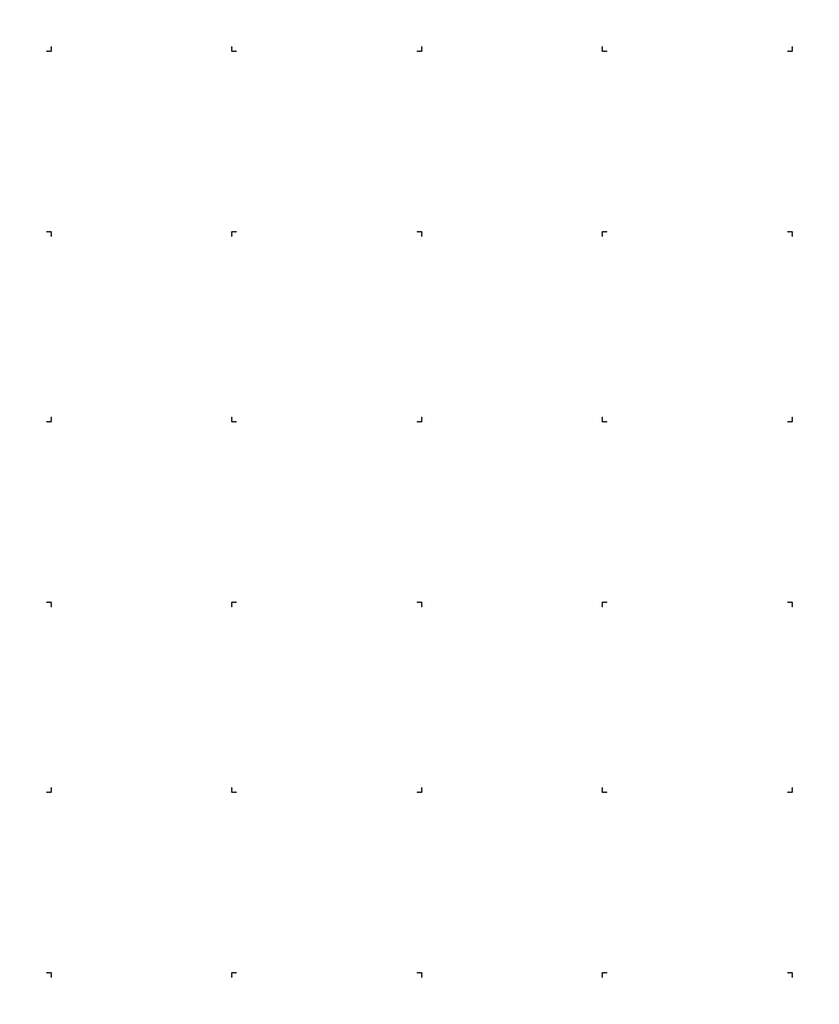
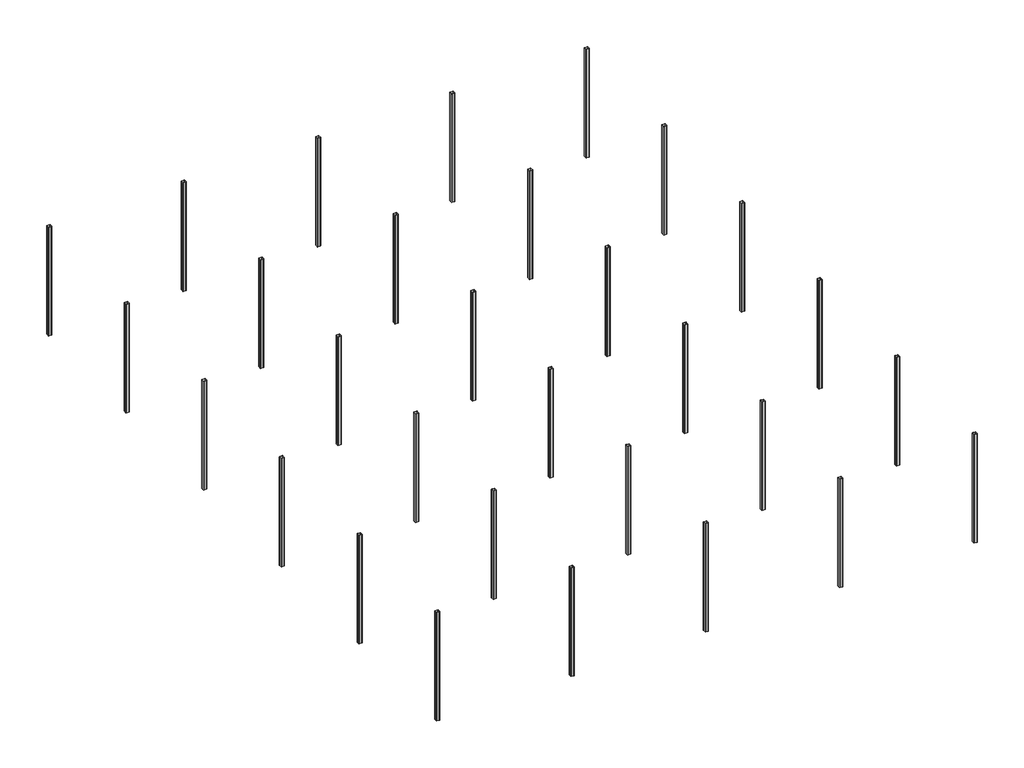
# One storey: 30 columns.
"""IFC4 building model written with IfcOpenShell, lengths in millimetres."""

import ifcopenshell
import ifcopenshell.guid

model = None  # the IFC model being written
_history = None  # IfcOwnerHistory: only IFC2X3 demands one
_inside = {}  # id of a spatial element -> (the spatial element, [elements in it])
_under = {}  # id of a project, library or spatial element -> (it, [spatial elements below it])
_declared = {}  # id of a project -> (the project, [libraries it declares])
_typed = {}  # id of a type object -> (the type object, [elements of that type])
_made_of = {}  # id of a material, layer set ... -> (it, [elements and type objects made of it])


def new_model(schema):
    """Start an empty IFC model of exactly this schema.

    Asked for "IFC4X3", IfcOpenShell would pick the latest addendum, in which some entities
    have other attributes; the version numbers below select the first issue.
    IFC2X3 requires an IfcOwnerHistory on every rooted entity: one is made here for all.
    """
    global model, _history
    if schema == "IFC4X3":
        model = ifcopenshell.file(schema_version=(4, 3, 0, 0))
    else:
        model = ifcopenshell.file(schema=schema)
    _inside.clear()
    _under.clear()
    _declared.clear()
    _typed.clear()
    _made_of.clear()
    _history = None
    if model.schema == "IFC2X3":
        org = make("IfcOrganization", Name="unknown")
        user = make(
            "IfcPersonAndOrganization",
            ThePerson=make("IfcPerson", FamilyName="unknown"),
            TheOrganization=org,
        )
        app = make(
            "IfcApplication",
            ApplicationDeveloper=org,
            Version="unknown",
            ApplicationFullName="unknown",
            ApplicationIdentifier="unknown",
        )
        _history = make(
            "IfcOwnerHistory",
            OwningUser=user,
            OwningApplication=app,
            ChangeAction="ADDED",
            CreationDate=0,
        )
    return model


def make(cls, **values):
    """One entity of the class cls with the attributes given. An attribute that is None is left unset."""
    return model.create_entity(
        cls, **{name: value for name, value in values.items() if value is not None}
    )


def rooted(cls, **values):
    """An entity with a GlobalId (a new one), such as an element, a storey or a relation."""
    return make(cls, GlobalId=ifcopenshell.guid.new(), OwnerHistory=_history, **values)


def si_unit(unit_type, name, prefix=None):
    """IfcSIUnit, for example si_unit("LENGTHUNIT", "METRE", prefix="MILLI")."""
    return make("IfcSIUnit", UnitType=unit_type, Prefix=prefix, Name=name)


def assignment(units):
    """IfcUnitAssignment: the units of a project."""
    return None if units is None else make("IfcUnitAssignment", Units=units)


def point(xyz):
    """IfcCartesianPoint."""
    return None if xyz is None else make("IfcCartesianPoint", Coordinates=xyz)


def direction(xyz):
    """IfcDirection."""
    return None if xyz is None else make("IfcDirection", DirectionRatios=xyz)


def frame(location, z_axis=None, x_axis=None):
    """IfcAxis2Placement3D, a coordinate frame: its origin and axes. An axis left out is left unset."""
    return make(
        "IfcAxis2Placement3D",
        Location=point(location),
        Axis=direction(z_axis),
        RefDirection=direction(x_axis),
    )


def frame_2d(location, x_axis=None):
    """IfcAxis2Placement2D, a coordinate frame in the plane: its origin and x axis."""
    return make(
        "IfcAxis2Placement2D", Location=point(location), RefDirection=direction(x_axis)
    )


def origin():
    """The frame at (0, 0, 0) with its axes left unset."""
    return frame((0.0, 0.0, 0.0))


def place(relative_to, where):
    """IfcLocalPlacement: puts the frame where relative to a parent placement (None: the world)."""
    return make(
        "IfcLocalPlacement", PlacementRelTo=relative_to, RelativePlacement=where
    )


def context(
    kind, dimensions, precision=None, world=None, true_north=None, identifier=None
):
    """IfcGeometricRepresentationContext, for example the 3D "Model" context."""
    return make(
        "IfcGeometricRepresentationContext",
        ContextIdentifier=identifier,
        ContextType=kind,
        CoordinateSpaceDimension=dimensions,
        Precision=precision,
        WorldCoordinateSystem=world,
        TrueNorth=true_north,
    )


def project(units=None, contexts=None):
    """IfcProject with its units and contexts."""
    return rooted(
        "IfcProject",
        Name="project",
        RepresentationContexts=contexts,
        UnitsInContext=assignment(units),
    )


def spatial(cls, under=None, at=None, **own):
    """A site, building, storey or space (cls), placed at a placement, below another one or the project."""
    s = rooted(cls, ObjectPlacement=at, **own)
    if under is not None:
        _under.setdefault(under.id(), (under, []))[1].append(s)
    return s


def polyline(points):
    """IfcPolyline through the points."""
    return make("IfcPolyline", Points=[point(p) for p in points])


def circle_curve(where, radius):
    """IfcCircle in the frame where."""
    return make("IfcCircle", Position=where, Radius=radius)


def trimmed(basis, trim1, trim2, sense, master):
    """IfcTrimmedCurve: the piece of a basis curve between two trims."""
    return make(
        "IfcTrimmedCurve",
        BasisCurve=basis,
        Trim1=trim1,
        Trim2=trim2,
        SenseAgreement=sense,
        MasterRepresentation=master,
    )


def segment(curve, same_sense, transition):
    """IfcCompositeCurveSegment."""
    return make(
        "IfcCompositeCurveSegment",
        Transition=transition,
        SameSense=same_sense,
        ParentCurve=curve,
    )


def composite_curve(segments, self_intersect=None):
    """IfcCompositeCurve: segments joined end to end."""
    return make("IfcCompositeCurve", Segments=segments, SelfIntersect=self_intersect)


def outline(outer, holes=None, kind="AREA"):
    """IfcArbitraryClosedProfileDef: a profile drawn as a closed curve; with holes, ...WithVoids."""
    if holes is None:
        return make("IfcArbitraryClosedProfileDef", ProfileType=kind, OuterCurve=outer)
    return make(
        "IfcArbitraryProfileDefWithVoids",
        ProfileType=kind,
        OuterCurve=outer,
        InnerCurves=holes,
    )


def extrude(swept, where, along, depth):
    """IfcExtrudedAreaSolid: the profile swept, set in the frame where, extruded along a direction by depth."""
    return make(
        "IfcExtrudedAreaSolid",
        SweptArea=swept,
        Position=where,
        ExtrudedDirection=direction(along),
        Depth=depth,
    )


def shape(context_of_items, identifier, shape_type, items):
    """IfcShapeRepresentation: the items that make up one representation, for example the "Body"."""
    return make(
        "IfcShapeRepresentation",
        ContextOfItems=context_of_items,
        RepresentationIdentifier=identifier,
        RepresentationType=shape_type,
        Items=items,
    )


def source(mapping_origin, context_of_items, identifier, shape_type, items):
    """IfcRepresentationMap: a shape defined once, which mapped items show again and again."""
    return make(
        "IfcRepresentationMap",
        MappingOrigin=mapping_origin,
        MappedRepresentation=shape(context_of_items, identifier, shape_type, items),
    )


def transform(
    local_origin,
    x_axis=None,
    y_axis=None,
    z_axis=None,
    scale=None,
    scale2=None,
    scale3=None,
    uniform=True,
):
    """IfcCartesianTransformationOperator3D, or its non-uniform kind. x_axis, y_axis, z_axis: its Axis1, 2, 3."""
    if uniform:
        return make(
            "IfcCartesianTransformationOperator3D",
            Axis1=direction(x_axis),
            Axis2=direction(y_axis),
            LocalOrigin=point(local_origin),
            Scale=scale,
            Axis3=direction(z_axis),
        )
    return make(
        "IfcCartesianTransformationOperator3DnonUniform",
        Axis1=direction(x_axis),
        Axis2=direction(y_axis),
        LocalOrigin=point(local_origin),
        Scale=scale,
        Axis3=direction(z_axis),
        Scale2=scale2,
        Scale3=scale3,
    )


def mapped(mapping_source, mapping_target):
    """IfcMappedItem: shows the shape of a source again, moved by a transform."""
    return make(
        "IfcMappedItem", MappingSource=mapping_source, MappingTarget=mapping_target
    )


def made_of(thing, what):
    """Note that an element or type object is made of a material, layer set ...; save() writes the relation."""
    if what is not None:
        _made_of.setdefault(what.id(), (what, []))[1].append(thing)
    return thing


def element(
    cls,
    number,
    at=None,
    inside=None,
    cuts=None,
    type_object=None,
    material=None,
    context=None,
    identifier="Body",
    shape_type=None,
    held_by="IfcProductDefinitionShape",
    body=None,
    shapes=None,
    **own,
):
    """One element of the class cls, such as IfcWall. Its Tag is "e" and its number.

    at: its placement. inside: the storey or other place that contains it. cuts: it is an
    opening in that element (IfcRelVoidsElement). A single representation is given by context,
    identifier, shape_type and body (its items); several are given by shapes. held_by: the class
    of the entity that holds the representations. save() writes the other relations.
    """
    e = rooted(cls, Tag="e%d" % number, ObjectPlacement=at, **own)
    if body is not None:
        shapes = [shape(context, identifier, shape_type, body)]
    if shapes is not None:
        e.Representation = make(held_by, Representations=shapes)
    if inside is not None:
        _inside.setdefault(inside.id(), (inside, []))[1].append(e)
    if cuts is not None:
        rooted(
            "IfcRelVoidsElement", RelatingBuildingElement=cuts, RelatedOpeningElement=e
        )
    if type_object is not None:
        _typed.setdefault(type_object.id(), (type_object, []))[1].append(e)
    return made_of(e, material)


def aggregate(whole, parts):
    """IfcRelAggregates: a whole, such as a stair, and the parts it consists of."""
    return rooted("IfcRelAggregates", RelatingObject=whole, RelatedObjects=parts)


def save(model, path):
    """Write the relations noted so far, then the file.

    IfcRelAggregates (storeys below a building ...), IfcRelContainedInSpatialStructure (elements
    in a storey), IfcRelDefinesByType, IfcRelAssociatesMaterial and IfcRelDeclares: one each for
    every whole, place, type object, material and project.
    """
    for whole, parts in _under.values():
        aggregate(whole, parts)
    for where, things in _inside.values():
        rooted(
            "IfcRelContainedInSpatialStructure",
            RelatedElements=things,
            RelatingStructure=where,
        )
    for kind, things in _typed.values():
        rooted("IfcRelDefinesByType", RelatedObjects=things, RelatingType=kind)
    for what, things in _made_of.values():
        rooted("IfcRelAssociatesMaterial", RelatedObjects=things, RelatingMaterial=what)
    for by, libraries in _declared.values():
        rooted("IfcRelDeclares", RelatingContext=by, RelatedDefinitions=libraries)
    model.write(path)


def pilar_quadrado_25x25_cm_e96a00db(model_context):
    return source(origin(), model_context, "Body", "SweptSolid", [
        extrude(outline(composite_curve([segment(trimmed(circle_curve(frame_2d((99.0, 99.0)), 26.0), [point((99.0, 125.0))], [point((125.0, 99.0))], False, "CARTESIAN"), True, "CONTINUOUS"), segment(polyline([(125.0, 99.0), (125.0, -99.0)]), True, "CONTINUOUS"), segment(trimmed(circle_curve(frame_2d((99.0, -99.0)), 26.0), [point((125.0, -99.0))], [point((99.0, -125.0))], False, "CARTESIAN"), True, "CONTINUOUS"), segment(polyline([(99.0, -125.0), (-99.0, -125.0)]), True, "CONTINUOUS"), segment(trimmed(circle_curve(frame_2d((-99.0, -99.0)), 26.0), [point((-99.0, -125.0))], [point((-125.0, -99.0))], False, "CARTESIAN"), True, "CONTINUOUS"), segment(polyline([(-125.0, -99.0), (-125.0, 99.0)]), True, "CONTINUOUS"), segment(trimmed(circle_curve(frame_2d((-99.0, 99.0)), 26.0), [point((-125.0, 99.0))], [point((-99.0, 125.0))], False, "CARTESIAN"), True, "CONTINUOUS"), segment(polyline([(-99.0, 125.0), (99.0, 125.0)]), True, "CONTINUOUS")], self_intersect=False), holes=[composite_curve([segment(polyline([(99.0, 112.0), (-99.0, 112.0)]), True, "CONTINUOUS"), segment(trimmed(circle_curve(frame_2d((-99.0, 99.0)), 13.0), [point((-99.0, 112.0))], [point((-112.0, 99.0))], True, "CARTESIAN"), True, "CONTINUOUS"), segment(polyline([(-112.0, 99.0), (-112.0, -99.0)]), True, "CONTINUOUS"), segment(trimmed(circle_curve(frame_2d((-99.0, -99.0)), 13.0), [point((-112.0, -99.0))], [point((-99.0, -112.0))], True, "CARTESIAN"), True, "CONTINUOUS"), segment(polyline([(-99.0, -112.0), (99.0, -112.0)]), True, "CONTINUOUS"), segment(trimmed(circle_curve(frame_2d((99.0, -99.0)), 13.0), [point((99.0, -112.0))], [point((112.0, -99.0))], True, "CARTESIAN"), True, "CONTINUOUS"), segment(polyline([(112.0, -99.0), (112.0, 99.0)]), True, "CONTINUOUS"), segment(trimmed(circle_curve(frame_2d((99.0, 99.0)), 13.0), [point((112.0, 99.0))], [point((99.0, 112.0))], True, "CARTESIAN"), True, "CONTINUOUS")], self_intersect=False)]), frame((0.0, 0.0, 39630.0), z_axis=(0.0, 0.0, 1.0), x_axis=(1.0, 0.0, 0.0)), (0.0, 0.0, 1.0), 8535.0),
    ])


model = new_model("IFC4")

# Units and contexts
model_context = context("Model", 3, world=origin())
ifc_project = project(units=[si_unit("LENGTHUNIT", "METRE", prefix="MILLI")], contexts=[model_context])

# Site, building, storey
site = spatial("IfcSite", under=ifc_project)
building = spatial("IfcBuilding", under=site)
storey = spatial("IfcBuildingStorey", under=building, Name="Nível TERRENO", Elevation=39630.0)

# Columns
placement = place(None, origin())
pilar_quadrado_25x25_cm_shape = pilar_quadrado_25x25_cm_e96a00db(model_context)
element("IfcColumn", 1, ObjectType="CEV-Corte da estrutura vazado-Coluna : pilar quadrado 25x25 cm", at=placement, inside=storey, context=model_context, shape_type="MappedRepresentation", body=[
    mapped(pilar_quadrado_25x25_cm_shape, transform((-11703.8168708, 12896.4376366, 0.0), x_axis=(1.0, 0.0, 0.0), y_axis=(0.0, 1.0, 0.0), z_axis=(0.0, 0.0, 1.0))),
])
element("IfcColumn", 2, ObjectType="CEV-Corte da estrutura vazado-Coluna : pilar quadrado 25x25 cm", at=placement, inside=storey, context=model_context, shape_type="MappedRepresentation", body=[
    mapped(pilar_quadrado_25x25_cm_shape, transform((-11703.8168708, 2896.4376366, 0.0), x_axis=(-1.0, 0.0, 0.0), y_axis=(0.0, -1.0, 0.0), z_axis=(0.0, 0.0, 1.0))),
])
element("IfcColumn", 3, ObjectType="CEV-Corte da estrutura vazado-Coluna : pilar quadrado 25x25 cm", at=placement, inside=storey, context=model_context, shape_type="MappedRepresentation", body=[
    mapped(pilar_quadrado_25x25_cm_shape, transform((-11703.8168708, -7103.5623634, 0.0), x_axis=(-1.0, 0.0, 0.0), y_axis=(0.0, -1.0, 0.0), z_axis=(0.0, 0.0, 1.0))),
])
element("IfcColumn", 4, ObjectType="CEV-Corte da estrutura vazado-Coluna : pilar quadrado 25x25 cm", at=placement, inside=storey, context=model_context, shape_type="MappedRepresentation", body=[
    mapped(pilar_quadrado_25x25_cm_shape, transform((-11703.8168708, -17103.5623634, 0.0), x_axis=(-1.0, 0.0, 0.0), y_axis=(0.0, -1.0, 0.0), z_axis=(0.0, 0.0, 1.0))),
])
element("IfcColumn", 5, ObjectType="CEV-Corte da estrutura vazado-Coluna : pilar quadrado 25x25 cm", at=placement, inside=storey, context=model_context, shape_type="MappedRepresentation", body=[
    mapped(pilar_quadrado_25x25_cm_shape, transform((-11703.8168708, -27103.5623634, 0.0), x_axis=(-1.0, 0.0, 0.0), y_axis=(0.0, -1.0, 0.0), z_axis=(0.0, 0.0, 1.0))),
])
element("IfcColumn", 6, ObjectType="CEV-Corte da estrutura vazado-Coluna : pilar quadrado 25x25 cm", at=placement, inside=storey, context=model_context, shape_type="MappedRepresentation", body=[
    mapped(pilar_quadrado_25x25_cm_shape, transform((-11703.8168708, -37103.5623634, 0.0), x_axis=(-1.0, 0.0, 0.0), y_axis=(0.0, -1.0, 0.0), z_axis=(0.0, 0.0, 1.0))),
])
element("IfcColumn", 7, ObjectType="CEV-Corte da estrutura vazado-Coluna : pilar quadrado 25x25 cm", at=placement, inside=storey, context=model_context, shape_type="MappedRepresentation", body=[
    mapped(pilar_quadrado_25x25_cm_shape, transform((-1703.8168708, 12896.4376366, 0.0), x_axis=(1.0, 0.0, 0.0), y_axis=(0.0, 1.0, 0.0), z_axis=(0.0, 0.0, 1.0))),
])
element("IfcColumn", 8, ObjectType="CEV-Corte da estrutura vazado-Coluna : pilar quadrado 25x25 cm", at=placement, inside=storey, context=model_context, shape_type="MappedRepresentation", body=[
    mapped(pilar_quadrado_25x25_cm_shape, transform((-1703.8168708, 2896.4376366, 0.0), x_axis=(-1.0, 0.0, 0.0), y_axis=(0.0, -1.0, 0.0), z_axis=(0.0, 0.0, 1.0))),
])
element("IfcColumn", 9, ObjectType="CEV-Corte da estrutura vazado-Coluna : pilar quadrado 25x25 cm", at=placement, inside=storey, context=model_context, shape_type="MappedRepresentation", body=[
    mapped(pilar_quadrado_25x25_cm_shape, transform((-1703.8168708, -7103.5623634, 0.0), x_axis=(-1.0, 0.0, 0.0), y_axis=(0.0, -1.0, 0.0), z_axis=(0.0, 0.0, 1.0))),
])
element("IfcColumn", 10, ObjectType="CEV-Corte da estrutura vazado-Coluna : pilar quadrado 25x25 cm", at=placement, inside=storey, context=model_context, shape_type="MappedRepresentation", body=[
    mapped(pilar_quadrado_25x25_cm_shape, transform((-1703.8168708, -17103.5623634, 0.0), x_axis=(-1.0, 0.0, 0.0), y_axis=(0.0, -1.0, 0.0), z_axis=(0.0, 0.0, 1.0))),
])
element("IfcColumn", 11, ObjectType="CEV-Corte da estrutura vazado-Coluna : pilar quadrado 25x25 cm", at=placement, inside=storey, context=model_context, shape_type="MappedRepresentation", body=[
    mapped(pilar_quadrado_25x25_cm_shape, transform((-1703.8168708, -27103.5623634, 0.0), x_axis=(-1.0, 0.0, 0.0), y_axis=(0.0, -1.0, 0.0), z_axis=(0.0, 0.0, 1.0))),
])
element("IfcColumn", 12, ObjectType="CEV-Corte da estrutura vazado-Coluna : pilar quadrado 25x25 cm", at=placement, inside=storey, context=model_context, shape_type="MappedRepresentation", body=[
    mapped(pilar_quadrado_25x25_cm_shape, transform((-1703.8168708, -37103.5623634, 0.0), x_axis=(-1.0, 0.0, 0.0), y_axis=(0.0, -1.0, 0.0), z_axis=(0.0, 0.0, 1.0))),
])
element("IfcColumn", 13, ObjectType="CEV-Corte da estrutura vazado-Coluna : pilar quadrado 25x25 cm", at=placement, inside=storey, context=model_context, shape_type="MappedRepresentation", body=[
    mapped(pilar_quadrado_25x25_cm_shape, transform((8296.1831292, 12896.4376366, 0.0), x_axis=(1.0, 0.0, 0.0), y_axis=(0.0, 1.0, 0.0), z_axis=(0.0, 0.0, 1.0))),
])
element("IfcColumn", 14, ObjectType="CEV-Corte da estrutura vazado-Coluna : pilar quadrado 25x25 cm", at=placement, inside=storey, context=model_context, shape_type="MappedRepresentation", body=[
    mapped(pilar_quadrado_25x25_cm_shape, transform((8296.1831292, 2896.4376366, 0.0), x_axis=(-1.0, 0.0, 0.0), y_axis=(0.0, -1.0, 0.0), z_axis=(0.0, 0.0, 1.0))),
])
element("IfcColumn", 15, ObjectType="CEV-Corte da estrutura vazado-Coluna : pilar quadrado 25x25 cm", at=placement, inside=storey, context=model_context, shape_type="MappedRepresentation", body=[
    mapped(pilar_quadrado_25x25_cm_shape, transform((8296.1831292, -7103.5623634, 0.0), x_axis=(-1.0, 0.0, 0.0), y_axis=(0.0, -1.0, 0.0), z_axis=(0.0, 0.0, 1.0))),
])
element("IfcColumn", 16, ObjectType="CEV-Corte da estrutura vazado-Coluna : pilar quadrado 25x25 cm", at=placement, inside=storey, context=model_context, shape_type="MappedRepresentation", body=[
    mapped(pilar_quadrado_25x25_cm_shape, transform((8296.1831292, -17103.5623634, 0.0), x_axis=(-1.0, 0.0, 0.0), y_axis=(0.0, -1.0, 0.0), z_axis=(0.0, 0.0, 1.0))),
])
element("IfcColumn", 17, ObjectType="CEV-Corte da estrutura vazado-Coluna : pilar quadrado 25x25 cm", at=placement, inside=storey, context=model_context, shape_type="MappedRepresentation", body=[
    mapped(pilar_quadrado_25x25_cm_shape, transform((8296.1831292, -27103.5623634, 0.0), x_axis=(-1.0, 0.0, 0.0), y_axis=(0.0, -1.0, 0.0), z_axis=(0.0, 0.0, 1.0))),
])
element("IfcColumn", 18, ObjectType="CEV-Corte da estrutura vazado-Coluna : pilar quadrado 25x25 cm", at=placement, inside=storey, context=model_context, shape_type="MappedRepresentation", body=[
    mapped(pilar_quadrado_25x25_cm_shape, transform((8296.1831292, -37103.5623634, 0.0), x_axis=(-1.0, 0.0, 0.0), y_axis=(0.0, -1.0, 0.0), z_axis=(0.0, 0.0, 1.0))),
])
element("IfcColumn", 19, ObjectType="CEV-Corte da estrutura vazado-Coluna : pilar quadrado 25x25 cm", at=placement, inside=storey, context=model_context, shape_type="MappedRepresentation", body=[
    mapped(pilar_quadrado_25x25_cm_shape, transform((18296.1831292, 12896.4376366, 0.0), x_axis=(1.0, 0.0, 0.0), y_axis=(0.0, 1.0, 0.0), z_axis=(0.0, 0.0, 1.0))),
])
element("IfcColumn", 20, ObjectType="CEV-Corte da estrutura vazado-Coluna : pilar quadrado 25x25 cm", at=placement, inside=storey, context=model_context, shape_type="MappedRepresentation", body=[
    mapped(pilar_quadrado_25x25_cm_shape, transform((18296.1831292, 2896.4376366, 0.0), x_axis=(-1.0, 0.0, 0.0), y_axis=(0.0, -1.0, 0.0), z_axis=(0.0, 0.0, 1.0))),
])
element("IfcColumn", 21, ObjectType="CEV-Corte da estrutura vazado-Coluna : pilar quadrado 25x25 cm", at=placement, inside=storey, context=model_context, shape_type="MappedRepresentation", body=[
    mapped(pilar_quadrado_25x25_cm_shape, transform((18296.1831292, -7103.5623634, 0.0), x_axis=(-1.0, 0.0, 0.0), y_axis=(0.0, -1.0, 0.0), z_axis=(0.0, 0.0, 1.0))),
])
element("IfcColumn", 22, ObjectType="CEV-Corte da estrutura vazado-Coluna : pilar quadrado 25x25 cm", at=placement, inside=storey, context=model_context, shape_type="MappedRepresentation", body=[
    mapped(pilar_quadrado_25x25_cm_shape, transform((18296.1831292, -17103.5623634, 0.0), x_axis=(-1.0, 0.0, 0.0), y_axis=(0.0, -1.0, 0.0), z_axis=(0.0, 0.0, 1.0))),
])
element("IfcColumn", 23, ObjectType="CEV-Corte da estrutura vazado-Coluna : pilar quadrado 25x25 cm", at=placement, inside=storey, context=model_context, shape_type="MappedRepresentation", body=[
    mapped(pilar_quadrado_25x25_cm_shape, transform((18296.1831292, -27103.5623634, 0.0), x_axis=(-1.0, 0.0, 0.0), y_axis=(0.0, -1.0, 0.0), z_axis=(0.0, 0.0, 1.0))),
])
element("IfcColumn", 24, ObjectType="CEV-Corte da estrutura vazado-Coluna : pilar quadrado 25x25 cm", at=placement, inside=storey, context=model_context, shape_type="MappedRepresentation", body=[
    mapped(pilar_quadrado_25x25_cm_shape, transform((18296.1831292, -37103.5623634, 0.0), x_axis=(-1.0, 0.0, 0.0), y_axis=(0.0, -1.0, 0.0), z_axis=(0.0, 0.0, 1.0))),
])
element("IfcColumn", 25, ObjectType="CEV-Corte da estrutura vazado-Coluna : pilar quadrado 25x25 cm", at=placement, inside=storey, context=model_context, shape_type="MappedRepresentation", body=[
    mapped(pilar_quadrado_25x25_cm_shape, transform((28296.1831292, 12896.4376366, 0.0), x_axis=(1.0, 0.0, 0.0), y_axis=(0.0, 1.0, 0.0), z_axis=(0.0, 0.0, 1.0))),
])
element("IfcColumn", 26, ObjectType="CEV-Corte da estrutura vazado-Coluna : pilar quadrado 25x25 cm", at=placement, inside=storey, context=model_context, shape_type="MappedRepresentation", body=[
    mapped(pilar_quadrado_25x25_cm_shape, transform((28296.1831292, 2896.4376366, 0.0), x_axis=(-1.0, 0.0, 0.0), y_axis=(0.0, -1.0, 0.0), z_axis=(0.0, 0.0, 1.0))),
])
element("IfcColumn", 27, ObjectType="CEV-Corte da estrutura vazado-Coluna : pilar quadrado 25x25 cm", at=placement, inside=storey, context=model_context, shape_type="MappedRepresentation", body=[
    mapped(pilar_quadrado_25x25_cm_shape, transform((28296.1831292, -7103.5623634, 0.0), x_axis=(-1.0, 0.0, 0.0), y_axis=(0.0, -1.0, 0.0), z_axis=(0.0, 0.0, 1.0))),
])
element("IfcColumn", 28, ObjectType="CEV-Corte da estrutura vazado-Coluna : pilar quadrado 25x25 cm", at=placement, inside=storey, context=model_context, shape_type="MappedRepresentation", body=[
    mapped(pilar_quadrado_25x25_cm_shape, transform((28296.1831292, -17103.5623634, 0.0), x_axis=(-1.0, 0.0, 0.0), y_axis=(0.0, -1.0, 0.0), z_axis=(0.0, 0.0, 1.0))),
])
element("IfcColumn", 29, ObjectType="CEV-Corte da estrutura vazado-Coluna : pilar quadrado 25x25 cm", at=placement, inside=storey, context=model_context, shape_type="MappedRepresentation", body=[
    mapped(pilar_quadrado_25x25_cm_shape, transform((28296.1831292, -27103.5623634, 0.0), x_axis=(-1.0, 0.0, 0.0), y_axis=(0.0, -1.0, 0.0), z_axis=(0.0, 0.0, 1.0))),
])
element("IfcColumn", 30, ObjectType="CEV-Corte da estrutura vazado-Coluna : pilar quadrado 25x25 cm", at=placement, inside=storey, context=model_context, shape_type="MappedRepresentation", body=[
    mapped(pilar_quadrado_25x25_cm_shape, transform((28296.1831292, -37103.5623634, 0.0), x_axis=(-1.0, 0.0, 0.0), y_axis=(0.0, -1.0, 0.0), z_axis=(0.0, 0.0, 1.0))),
])

save(model, "model.ifc")

# Revit data of these elements
# Project information
#   Data de emissão do projeto = "Data de emissão"
#   Status do projeto = "Status do projeto"
#   Nome do cliente = "Proprietário"
#   Endereço do projeto = "Enter address here"
#   Nome do projeto = "Nome do projeto"
#   Número do projeto = "0001"
# Grids (mm)
#   "3": line (-11703.817, -42662.286) -> (-11703.817, 17514.974)
#   "4": line (-1703.817, -42662.286) -> (-1703.817, 17514.974)
#   "5": line (8296.183, -42662.286) -> (8296.183, 17514.974)
#   "6": line (18296.183, -42662.286) -> (18296.183, 17514.974)
#   "A": line (32919.939, 12896.438) -> (-20751.533, 12896.438)
#   "B": line (-20751.533, 2896.438) -> (32919.939, 2896.438)
#   "C": line (-20751.533, -7103.562) -> (32919.939, -7103.562)
#   "D": line (-20751.533, -17103.562) -> (32919.939, -17103.562)
#   "E": line (-20751.533, -27103.562) -> (32919.939, -27103.562)
#   "F": line (-20751.533, -37103.562) -> (32919.939, -37103.562)
#   "7": line (28296.183, 17514.974) -> (28296.183, -42662.286)
# Type "CEV-Corte da estrutura vazado-Coluna : pilar quadrado 25x25 cm"
#   Forma = "Quadrado"
#   W = 0.0258
#   Ht = 0.25 m
#   b = 0.25 m
#   kr = 0.026 m
#   t = 0.013 m
#   A = 0.000317 m²
#   Structural Material [instance default] = Aço, 45-345
#   Assembly Code = ""
# Elements 1, 2, 3, 4, 5, 6, 7, 8, 9, 10, 11, 12, 13, 14, 15, 16, 17, 18, 19, 20, 21, 22, 23, 24, 25, 26, 27, 28, 29, 30 (IfcColumn, "CEV-Corte da estrutura vazado-Coluna : pilar quadrado 25x25 cm")
#   Structural Material = Aço, 45-345
#   Phase Created = Construção nova
#   Materials on its faces: "Aço, 45-345"
# Materials
#   "Aço, 45-345": class "Metal", colour RGB 247 247 247, transparency 0, Description = "Aço 345 MPa", Cost = 0
